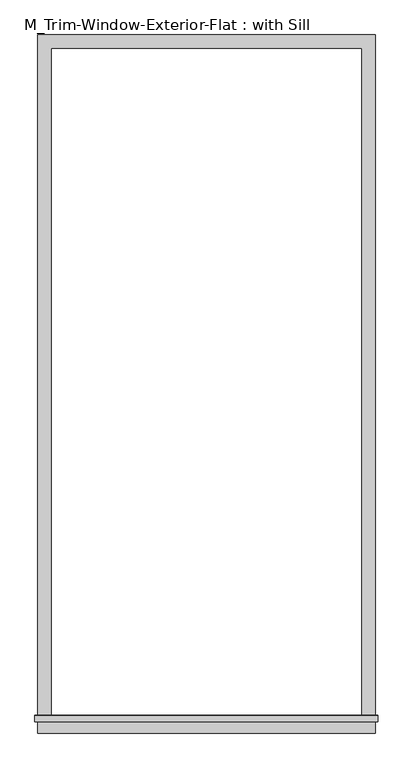
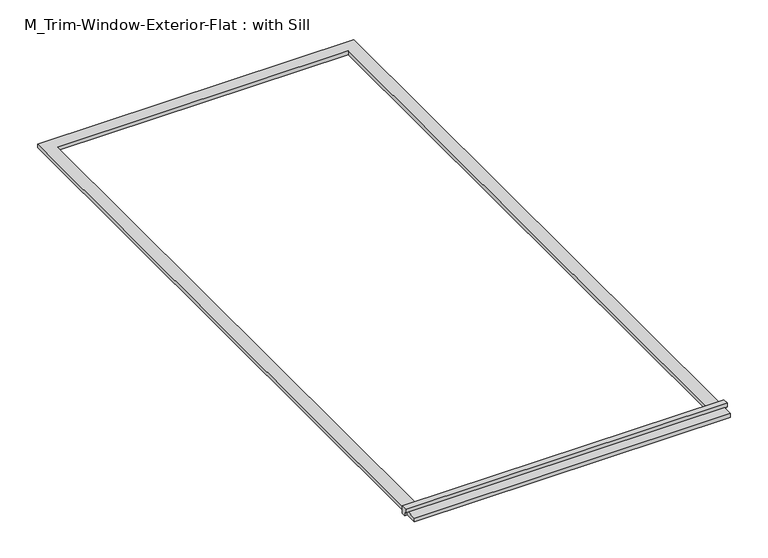
"""IFC4 building model written with IfcOpenShell, lengths in millimetres: proxy geometry, M_Trim-Window-Exterior-Flat : with Sill."""

from ifc_helpers import new_model, si_unit, frame, origin, origin_with_axes, place, context, project, spatial, polyline, outline, extrude, source, transform, mapped, element, save


def m_trim_window_exterior_flat_with_sill_aad1028e(model_context):
    return source(origin(), model_context, "Body", "SweptSolid", [
        extrude(outline(polyline([(760.0, -3020.4323709), (760.0, -3080.4323709), (-760.0, -3080.4323709), (-760.0, -3020.4323709), (760.0, -3020.4323709)])), origin_with_axes(), (0.0, 0.0, 1.0), 19.05),
        extrude(outline(polyline([(-3030.0, 38.1), (-3002.4580645, 38.1), (-3000.0, 19.05), (-3000.0, 0.0), (-3020.4323709, 0.0), (-3020.4323709, 19.05), (-3030.0, 19.05), (-3030.0, 38.1)])), frame((-772.7, 0.0, 0.0), z_axis=(1.0, 0.0, 0.0), x_axis=(0.0, 1.0, 0.0)), (0.0, 0.0, 1.0), 1545.4),
        extrude(outline(polyline([(-760.0, 60.0), (760.0, 60.0), (760.0, -3000.0), (700.0, -3000.0), (700.0, 0.0), (-700.0, 0.0), (-700.0, -3000.0), (-760.0, -3000.0), (-760.0, 60.0)])), origin_with_axes(), (0.0, 0.0, 1.0), 19.05),
    ])


if __name__ == "__main__":
    model = new_model("IFC4")
    model_context = context("Model", 3, world=origin())
    ifc_project = project(units=[si_unit("LENGTHUNIT", "METRE", prefix="MILLI")], contexts=[model_context])
    site = spatial("IfcSite", under=ifc_project)
    building = spatial("IfcBuilding", under=site)
    placement = place(None, origin())
    m_trim_window_exterior_flat_with_sill_shape = m_trim_window_exterior_flat_with_sill_aad1028e(model_context)
    element("IfcBuildingElementProxy", 1, Name="M_Trim-Window-Exterior-Flat : with Sill", ObjectType="M_Trim-Window-Exterior-Flat : with Sill", at=placement, inside=building, context=model_context, shape_type="MappedRepresentation", body=[
        mapped(m_trim_window_exterior_flat_with_sill_shape, transform((0.0, 0.0, 0.0), x_axis=(1.0, 0.0, 0.0), y_axis=(0.0, 1.0, 0.0), z_axis=(0.0, 0.0, 1.0))),
    ])
    save(model, "model.ifc")

# Revit data of these elements
# Type "M_Trim-Window-Exterior-Flat : with Sill"
#   Trim Width = 60 mm
#   Trim Thickness_Picture Frame = 30 mm
#   Trim Thickness_with Sill = 19.05 mm
#   Sill Thickness = 30 mm
#   Opening Width [instance default] = 600 mm
#   Opening Height [instance default] = 900 mm
#   Default Elevation = 1200 mm
#   Sill = yes
#   Picture Frame = no
#   Trim Material [instance default] = none
# Element 1 (IfcBuildingElementProxy, "M_Trim-Window-Exterior-Flat : with Sill")
#   Opening Width = 1400 mm
#   Opening Height = 3000 mm
#   Trim Material = Clad - White
#   Materials on its faces: "Clad - White"
# Materials
#   "Clad - White": class "Wood", colour RGB 245 245 243, transparency 0, Cost = 0
